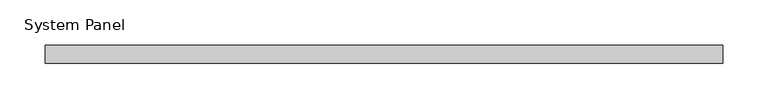
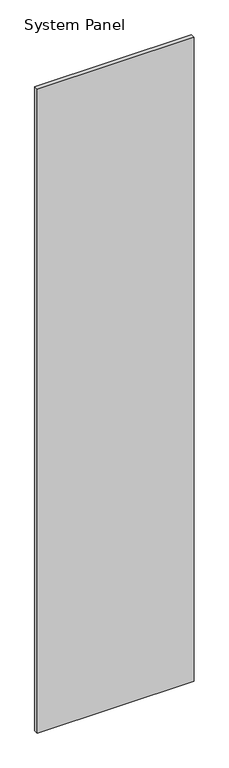
"""IFC4 building model written with IfcOpenShell, lengths in millimetres: plate geometry, System Panel : WWm-Glass-20mm-10mmOffset."""

from ifc_helpers import new_model, si_unit, origin, origin_with_axes, place, context, project, spatial, polyline, outline, extrude, source, transform, mapped, element, save


def system_panel_35fc1531(model_context):
    return source(origin(), model_context, "Body", "SweptSolid", [
        extrude(outline(polyline([(375.0, 0.0), (-375.0, 0.0), (-375.0, 20.0), (375.0, 20.0), (375.0, 0.0)])), origin_with_axes(), (0.0, 0.0, 1.0), 3250.0),
    ])


if __name__ == "__main__":
    model = new_model("IFC4")
    model_context = context("Model", 3, world=origin())
    ifc_project = project(units=[si_unit("LENGTHUNIT", "METRE", prefix="MILLI")], contexts=[model_context])
    site = spatial("IfcSite", under=ifc_project)
    building = spatial("IfcBuilding", under=site)
    placement = place(None, origin())
    system_panel_shape = system_panel_35fc1531(model_context)
    element("IfcPlate", 1, ObjectType="System Panel : WWm-Glass-20mm-10mmOffset", at=placement, inside=building, context=model_context, shape_type="MappedRepresentation", body=[
        mapped(system_panel_shape, transform((0.0, 0.0, 0.0), x_axis=(1.0, 0.0, 0.0), y_axis=(0.0, 1.0, 0.0), z_axis=(0.0, 0.0, 1.0))),
    ])
    save(model, "model.ifc")

# Revit data of these elements
# Type "System Panel : WWm-Glass-20mm-10mmOffset"
#   Finish = ""
# Element 1 (IfcPlate, "System Panel : WWm-Glass-20mm-10mmOffset")
#   Materials on its faces: "WW-EC-GL-Storefront"
# Materials
#   "WW-EC-GL-Storefront": class "Glass", colour RGB 236 240 239, transparency 0.85, Description = "Storefront Glass", Cost = 0
